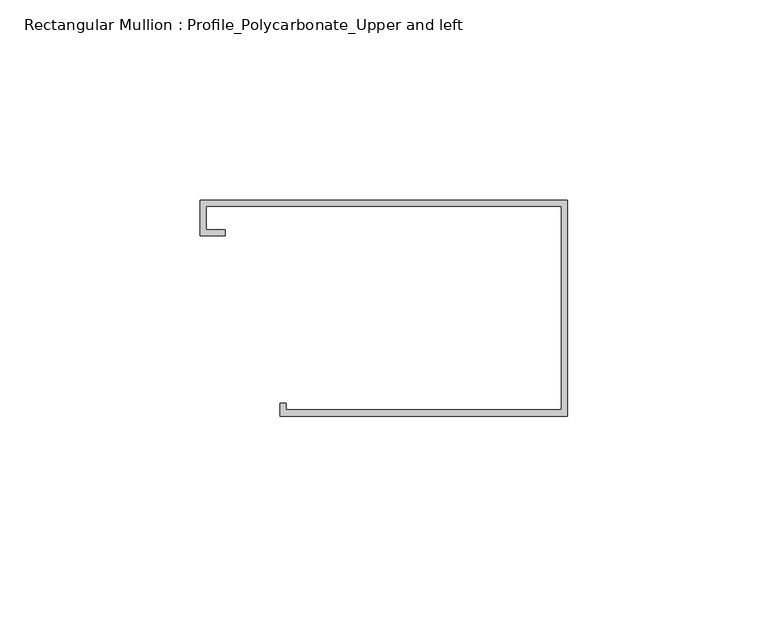
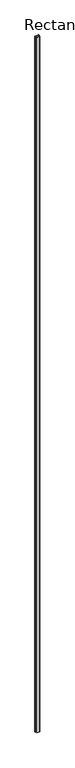
"""IFC4 building model written with IfcOpenShell, lengths in millimetres: member geometry, Rectangular Mullion : Profile_Polycarbonate_Upper and left."""

from ifc_helpers import new_model, si_unit, frame, origin, place, context, project, spatial, polyline, outline, extrude, source, transform, mapped, element, save


def rectangular_mullion_profile_polycarbonate_upper_and_left_0c3de010(model_context):
    return source(origin(), model_context, "Body", "SweptSolid", [
        extrude(outline(polyline([(0.0, 28.984575), (0.0, -25.015825), (-71.9836, -25.015825), (-71.9836, -21.840825), (-70.3961, -21.840825), (-70.3961, -23.428325), (-1.5875, -23.428325), (-1.5875, 27.397075), (-90.4113, 27.397075), (-90.4113, 21.580475), (-85.6488, 21.580475), (-85.6488, 19.992975), (-91.9988, 19.992975), (-91.9988, 28.984575), (0.0, 28.984575)])), frame((0.0, 0.0, -18548.5024), z_axis=(0.0, 0.0, 1.0), x_axis=(1.0, 0.0, 0.0)), (0.0, 0.0, 1.0), 18548.5024),
    ])


if __name__ == "__main__":
    model = new_model("IFC4")
    model_context = context("Model", 3, world=origin())
    ifc_project = project(units=[si_unit("LENGTHUNIT", "METRE", prefix="MILLI")], contexts=[model_context])
    site = spatial("IfcSite", under=ifc_project)
    building = spatial("IfcBuilding", under=site)
    placement = place(None, origin())
    rectangular_mullion_profile_polycarbonate_upper_and_left_shape = rectangular_mullion_profile_polycarbonate_upper_and_left_0c3de010(model_context)
    element("IfcMember", 1, ObjectType="Rectangular Mullion : Profile_Polycarbonate_Upper and left", at=placement, inside=building, context=model_context, shape_type="MappedRepresentation", body=[
        mapped(rectangular_mullion_profile_polycarbonate_upper_and_left_shape, transform((0.0, 0.0, 0.0), x_axis=(1.0, 0.0, 0.0), y_axis=(0.0, 1.0, 0.0), z_axis=(0.0, 0.0, 1.0))),
    ])
    save(model, "model.ifc")

# Revit data of these elements
# Type "Rectangular Mullion : Profile_Polycarbonate_Upper and left"
#   built-in parameter 1007322 = 0.177167 (stored number, unit not read)
#   built-in parameter 1007321 = 0.00520833 (stored number, unit not read)
#   built-in parameter 1007320 = 0 (stored number, unit not read)
